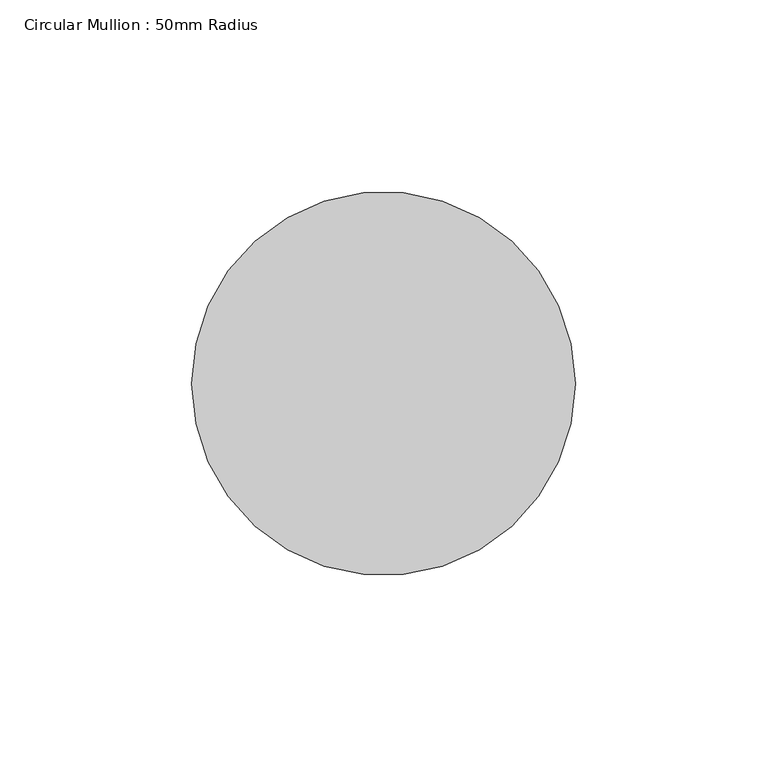
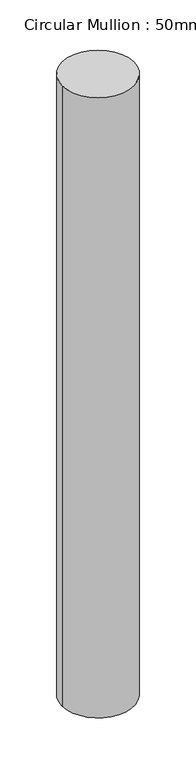
"""IFC4 building model written with IfcOpenShell, lengths in millimetres: member geometry, Circular Mullion : 50mm Radius."""

from ifc_helpers import new_model, si_unit, point, frame, origin, origin_2d, place, context, project, spatial, circle_curve, trimmed, segment, composite_curve, outline, extrude, source, transform, mapped, element, save


def circular_mullion_50mm_radius_6f459f22(model_context):
    return source(origin(), model_context, "Body", "SweptSolid", [
        extrude(outline(composite_curve([segment(trimmed(circle_curve(origin_2d(), 50.0), [point((50.0, 0.0))], [point((-50.0, 0.0))], False, "CARTESIAN"), True, "CONTINUOUS"), segment(trimmed(circle_curve(origin_2d(), 50.0), [point((-50.0, 0.0))], [point((50.0, 0.0))], False, "CARTESIAN"), True, "CONTINUOUS")], self_intersect=False)), frame((0.0, 0.0, -914.9278018), z_axis=(0.0, 0.0, 1.0), x_axis=(1.0, 0.0, 0.0)), (0.0, 0.0, 1.0), 914.9278018),
    ])


if __name__ == "__main__":
    model = new_model("IFC4")
    model_context = context("Model", 3, world=origin())
    ifc_project = project(units=[si_unit("LENGTHUNIT", "METRE", prefix="MILLI")], contexts=[model_context])
    site = spatial("IfcSite", under=ifc_project)
    building = spatial("IfcBuilding", under=site)
    placement = place(None, origin())
    circular_mullion_50mm_radius_shape = circular_mullion_50mm_radius_6f459f22(model_context)
    element("IfcMember", 1, ObjectType="Circular Mullion : 50mm Radius", at=placement, inside=building, context=model_context, shape_type="MappedRepresentation", body=[
        mapped(circular_mullion_50mm_radius_shape, transform((0.0, 0.0, 0.0), x_axis=(1.0, 0.0, 0.0), y_axis=(0.0, 1.0, 0.0), z_axis=(0.0, 0.0, 1.0))),
    ])
    save(model, "model.ifc")

# Revit data of these elements
# Type "Circular Mullion : 50mm Radius"
#   built-in parameter 1007350 = 0.164042 (stored number, unit not read)
# Element 1 (IfcMember, "Circular Mullion : 50mm Radius")
#   Materials on its faces: "Aluminium"
# Materials
#   "Aluminium": class "Metal", colour RGB 247 247 247, transparency 0, Description = "Aluminium 6061", Cost = 0
